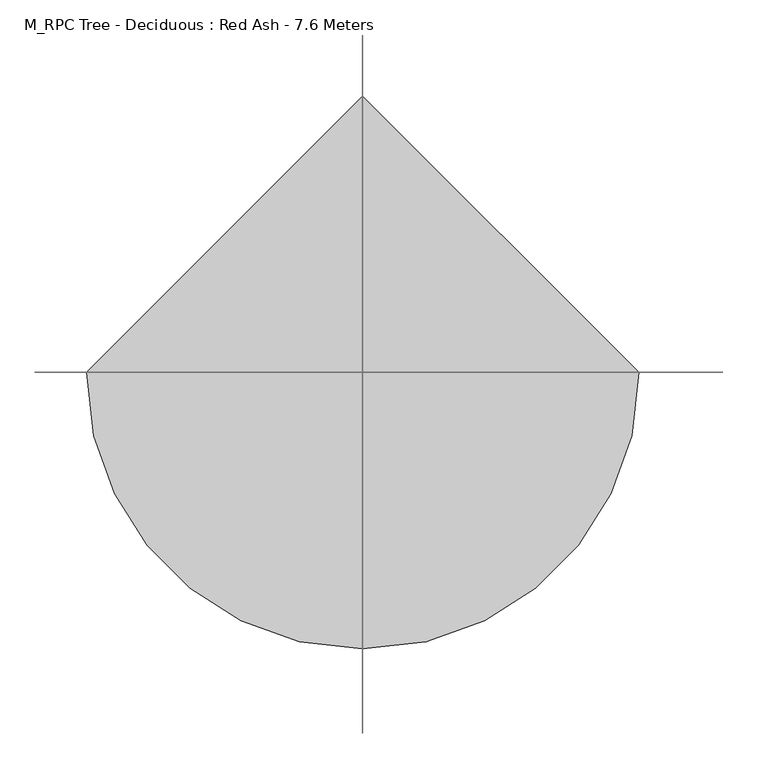
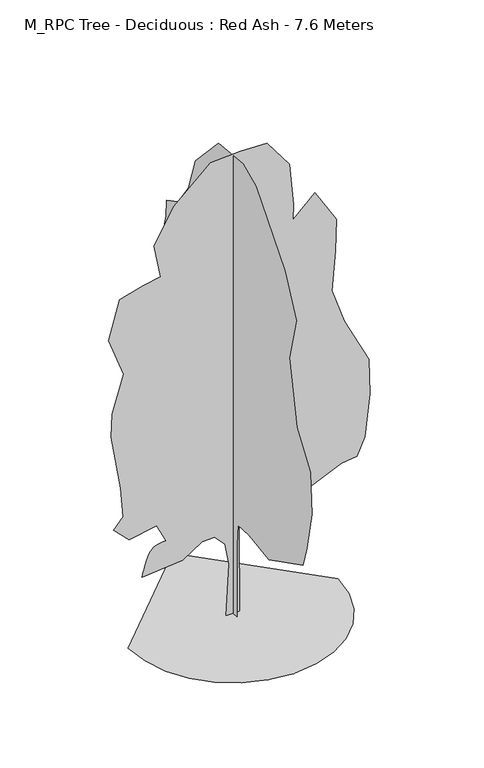
"""IFC4 building model written with IfcOpenShell, lengths in millimetres: geographic element geometry, M_RPC Tree - Deciduous : Red Ash - 7.6 Meters."""

import ifcopenshell
import ifcopenshell.guid

model = None  # the IFC model being written
_history = None  # IfcOwnerHistory: only IFC2X3 demands one
_inside = {}  # id of a spatial element -> (the spatial element, [elements in it])
_under = {}  # id of a project, library or spatial element -> (it, [spatial elements below it])
_declared = {}  # id of a project -> (the project, [libraries it declares])
_typed = {}  # id of a type object -> (the type object, [elements of that type])
_made_of = {}  # id of a material, layer set ... -> (it, [elements and type objects made of it])


def new_model(schema):
    """Start an empty IFC model of exactly this schema.

    Asked for "IFC4X3", IfcOpenShell would pick the latest addendum, in which some entities
    have other attributes; the version numbers below select the first issue.
    IFC2X3 requires an IfcOwnerHistory on every rooted entity: one is made here for all.
    """
    global model, _history
    if schema == "IFC4X3":
        model = ifcopenshell.file(schema_version=(4, 3, 0, 0))
    else:
        model = ifcopenshell.file(schema=schema)
    _inside.clear()
    _under.clear()
    _declared.clear()
    _typed.clear()
    _made_of.clear()
    _history = None
    if model.schema == "IFC2X3":
        org = make("IfcOrganization", Name="unknown")
        user = make(
            "IfcPersonAndOrganization",
            ThePerson=make("IfcPerson", FamilyName="unknown"),
            TheOrganization=org,
        )
        app = make(
            "IfcApplication",
            ApplicationDeveloper=org,
            Version="unknown",
            ApplicationFullName="unknown",
            ApplicationIdentifier="unknown",
        )
        _history = make(
            "IfcOwnerHistory",
            OwningUser=user,
            OwningApplication=app,
            ChangeAction="ADDED",
            CreationDate=0,
        )
    return model


def make(cls, **values):
    """One entity of the class cls with the attributes given. An attribute that is None is left unset."""
    return model.create_entity(
        cls, **{name: value for name, value in values.items() if value is not None}
    )


def rooted(cls, **values):
    """An entity with a GlobalId (a new one), such as an element, a storey or a relation."""
    return make(cls, GlobalId=ifcopenshell.guid.new(), OwnerHistory=_history, **values)


def si_unit(unit_type, name, prefix=None):
    """IfcSIUnit, for example si_unit("LENGTHUNIT", "METRE", prefix="MILLI")."""
    return make("IfcSIUnit", UnitType=unit_type, Prefix=prefix, Name=name)


def assignment(units):
    """IfcUnitAssignment: the units of a project."""
    return None if units is None else make("IfcUnitAssignment", Units=units)


def point(xyz):
    """IfcCartesianPoint."""
    return None if xyz is None else make("IfcCartesianPoint", Coordinates=xyz)


def direction(xyz):
    """IfcDirection."""
    return None if xyz is None else make("IfcDirection", DirectionRatios=xyz)


def frame(location, z_axis=None, x_axis=None):
    """IfcAxis2Placement3D, a coordinate frame: its origin and axes. An axis left out is left unset."""
    return make(
        "IfcAxis2Placement3D",
        Location=point(location),
        Axis=direction(z_axis),
        RefDirection=direction(x_axis),
    )


def origin():
    """The frame at (0, 0, 0) with its axes left unset."""
    return frame((0.0, 0.0, 0.0))


def place(relative_to, where):
    """IfcLocalPlacement: puts the frame where relative to a parent placement (None: the world)."""
    return make(
        "IfcLocalPlacement", PlacementRelTo=relative_to, RelativePlacement=where
    )


def context(
    kind, dimensions, precision=None, world=None, true_north=None, identifier=None
):
    """IfcGeometricRepresentationContext, for example the 3D "Model" context."""
    return make(
        "IfcGeometricRepresentationContext",
        ContextIdentifier=identifier,
        ContextType=kind,
        CoordinateSpaceDimension=dimensions,
        Precision=precision,
        WorldCoordinateSystem=world,
        TrueNorth=true_north,
    )


def project(units=None, contexts=None):
    """IfcProject with its units and contexts."""
    return rooted(
        "IfcProject",
        Name="project",
        RepresentationContexts=contexts,
        UnitsInContext=assignment(units),
    )


def spatial(cls, under=None, at=None, **own):
    """A site, building, storey or space (cls), placed at a placement, below another one or the project."""
    s = rooted(cls, ObjectPlacement=at, **own)
    if under is not None:
        _under.setdefault(under.id(), (under, []))[1].append(s)
    return s


def point_list(points):
    """IfcCartesianPointList2D or 3D."""
    cls = (
        "IfcCartesianPointList2D" if len(points[0]) == 2 else "IfcCartesianPointList3D"
    )
    return make(cls, CoordList=points)


def triangles(points, corners, closed=None, point_numbers=None):
    """IfcTriangulatedFaceSet: each triangle names its three corners, points numbered from 1."""
    return make(
        "IfcTriangulatedFaceSet",
        Coordinates=point_list(points),
        Closed=closed,
        CoordIndex=corners,
        PnIndex=point_numbers,
    )


def shape(context_of_items, identifier, shape_type, items):
    """IfcShapeRepresentation: the items that make up one representation, for example the "Body"."""
    return make(
        "IfcShapeRepresentation",
        ContextOfItems=context_of_items,
        RepresentationIdentifier=identifier,
        RepresentationType=shape_type,
        Items=items,
    )


def source(mapping_origin, context_of_items, identifier, shape_type, items):
    """IfcRepresentationMap: a shape defined once, which mapped items show again and again."""
    return make(
        "IfcRepresentationMap",
        MappingOrigin=mapping_origin,
        MappedRepresentation=shape(context_of_items, identifier, shape_type, items),
    )


def transform(
    local_origin,
    x_axis=None,
    y_axis=None,
    z_axis=None,
    scale=None,
    scale2=None,
    scale3=None,
    uniform=True,
):
    """IfcCartesianTransformationOperator3D, or its non-uniform kind. x_axis, y_axis, z_axis: its Axis1, 2, 3."""
    if uniform:
        return make(
            "IfcCartesianTransformationOperator3D",
            Axis1=direction(x_axis),
            Axis2=direction(y_axis),
            LocalOrigin=point(local_origin),
            Scale=scale,
            Axis3=direction(z_axis),
        )
    return make(
        "IfcCartesianTransformationOperator3DnonUniform",
        Axis1=direction(x_axis),
        Axis2=direction(y_axis),
        LocalOrigin=point(local_origin),
        Scale=scale,
        Axis3=direction(z_axis),
        Scale2=scale2,
        Scale3=scale3,
    )


def mapped(mapping_source, mapping_target):
    """IfcMappedItem: shows the shape of a source again, moved by a transform."""
    return make(
        "IfcMappedItem", MappingSource=mapping_source, MappingTarget=mapping_target
    )


def made_of(thing, what):
    """Note that an element or type object is made of a material, layer set ...; save() writes the relation."""
    if what is not None:
        _made_of.setdefault(what.id(), (what, []))[1].append(thing)
    return thing


def element(
    cls,
    number,
    at=None,
    inside=None,
    cuts=None,
    type_object=None,
    material=None,
    context=None,
    identifier="Body",
    shape_type=None,
    held_by="IfcProductDefinitionShape",
    body=None,
    shapes=None,
    **own,
):
    """One element of the class cls, such as IfcWall. Its Tag is "e" and its number.

    at: its placement. inside: the storey or other place that contains it. cuts: it is an
    opening in that element (IfcRelVoidsElement). A single representation is given by context,
    identifier, shape_type and body (its items); several are given by shapes. held_by: the class
    of the entity that holds the representations. save() writes the other relations.
    """
    e = rooted(cls, Tag="e%d" % number, ObjectPlacement=at, **own)
    if body is not None:
        shapes = [shape(context, identifier, shape_type, body)]
    if shapes is not None:
        e.Representation = make(held_by, Representations=shapes)
    if inside is not None:
        _inside.setdefault(inside.id(), (inside, []))[1].append(e)
    if cuts is not None:
        rooted(
            "IfcRelVoidsElement", RelatingBuildingElement=cuts, RelatedOpeningElement=e
        )
    if type_object is not None:
        _typed.setdefault(type_object.id(), (type_object, []))[1].append(e)
    return made_of(e, material)


def aggregate(whole, parts):
    """IfcRelAggregates: a whole, such as a stair, and the parts it consists of."""
    return rooted("IfcRelAggregates", RelatingObject=whole, RelatedObjects=parts)


def save(model, path):
    """Write the relations noted so far, then the file.

    IfcRelAggregates (storeys below a building ...), IfcRelContainedInSpatialStructure (elements
    in a storey), IfcRelDefinesByType, IfcRelAssociatesMaterial and IfcRelDeclares: one each for
    every whole, place, type object, material and project.
    """
    for whole, parts in _under.values():
        aggregate(whole, parts)
    for where, things in _inside.values():
        rooted(
            "IfcRelContainedInSpatialStructure",
            RelatedElements=things,
            RelatingStructure=where,
        )
    for kind, things in _typed.values():
        rooted("IfcRelDefinesByType", RelatedObjects=things, RelatingType=kind)
    for what, things in _made_of.values():
        rooted("IfcRelAssociatesMaterial", RelatedObjects=things, RelatingMaterial=what)
    for by, libraries in _declared.values():
        rooted("IfcRelDeclares", RelatingContext=by, RelatedDefinitions=libraries)
    model.write(path)


def m_rpc_tree_deciduous_red_ash_7_6_meters_16c8020d(model_context):
    return source(origin(), model_context, "Body", "Tessellation", [
        triangles([(-1640.6350319, 0.0, 6.17e-05), (-1597.2618073, -375.9250554, 6.17e-05), (-1473.7362076, -721.1521299, 6.17e-05), (-1279.9481815, -1025.7899305, 6.17e-05), (-1025.7900759, -1279.9483269, 6.17e-05), (-721.1519119, -1473.7357716, 6.17e-05), (-375.9249101, -1597.2618073, 6.17e-05), (7.17e-05, -1640.6350319, 6.17e-05), (375.9250917, -1597.2619526, 6.17e-05), (721.1521299, -1473.7360622, 6.17e-05), (1025.7900759, -1279.9481815, 6.17e-05), (1279.9486176, -1025.7900759, 6.17e-05), (1473.7359169, -721.1518393, 6.17e-05), (1597.2618073, -375.9248011, 6.17e-05), (1640.6350319, 0.0001434, 6.17e-05), (-0.0002151, 1640.6350319, 6.17e-05), (-1.07e-05, -102.5763152, 0.0), (2.5e-05, -100.9809819, 1191.4187742), (3.22e-05, -129.5410573, 1533.7667004), (7e-07, -437.6736119, 1554.0757805), (-5.76e-05, -973.8285673, 1474.4268631), (-0.0001401, -1898.6961697, 1943.5624718), (-0.0001409, -2005.9272697, 2292.063438), (-0.0001357, -2139.9660358, 2935.4493118), (-0.0001116, -2099.7546822, 3605.6435783), (-5.8e-05, -1735.814106, 4130.1484818), (-5.5e-06, -1523.3897175, 5147.0898972), (-3.5e-06, -1711.0423622, 5870.899205), (4.78e-05, -1402.7536217, 6514.2855148), (0.0001565, -625.3287638, 7439.1534805), (0.000198, -272.4836404, 7598.1990051), (0.0002655, 393.3664327, 7532.9808929), (0.0003113, 1023.3488731, 6862.7869171), (0.0003141, 1211.0034073, 6299.8236053), (0.0003314, 1492.4837551, 5897.706871), (0.0003588, 1800.7742397, 5736.8608749), (0.0003522, 1814.1780727, 5468.7830521), (0.0003514, 1894.6015068, 5160.4937302), (0.0003267, 1760.5627407, 4798.5890762), (0.0003288, 1881.1975285, 4450.088546), (0.000327, 2001.8324615, 3967.5488136), (0.0003203, 1975.0247955, 3833.5096115), (0.0002869, 1747.159053, 3511.8164566), (0.0002722, 1732.7516476, 3069.4885139), (0.0002625, 1720.3510963, 2788.0068581), (0.0002535, 1733.7549294, 2439.5063278), (0.0002406, 1747.159053, 1956.9668861), (0.0002166, 1559.5045189, 1809.523851), (0.0001802, 1211.0038433, 1809.523851), (0.0001822, 1371.8504208, 1313.580431), (0.0001711, 1344.9556961, 1032.1683203), (0.0001512, 1100.1359739, 1224.6137684), (9.84e-05, 627.810589, 1103.8028286), (9.77e-05, 550.2637599, 1353.49907), (6.27e-05, 215.346067, 1350.4488201), (5.01e-05, 130.4579254, 1225.1105404), (3.26e-05, 79.3405423, 816.1354311), (1.17e-05, 111.8716144, 1.28e-05), (-110.5798692, 4.8e-06, 4.45e-05), (-66.5363775, -9.62e-05, 831.3140104), (-128.9679092, -0.0001356, 1184.825572), (-290.0246482, -0.0001497, 1361.7341778), (-482.3670685, -0.0001405, 1355.1302204), (-794.1778324, -0.0001027, 1152.7338535), (-1424.1601639, -6.88e-05, 1099.1184488), (-1415.4458702, -7.33e-05, 1133.7810133), (-1406.1451298, -7.8e-05, 1169.6158899), (-1395.6722225, -8.3e-05, 1207.7952456), (-1383.4407017, -8.85e-05, 1249.4921917), (-1368.8645565, -9.46e-05, 1295.8774418), (-1351.3574856, -0.0001016, 1348.1257061), (-1330.3333328, -0.0001096, 1407.4074074), (-1303.8382931, -0.0001173, 1462.3908245), (-1271.0123898, -0.0001236, 1502.6024689), (-1232.9109364, -0.0001286, 1530.5039635), (-1190.588883, -0.0001326, 1548.5586754), (-1145.1018339, -0.0001358, 1559.2267742), (-1097.5041578, -0.0001386, 1564.971191), (-1048.8515316, -0.0001411, 1568.2539848), (-1196.294058, -0.0001698, 1863.1393284), (-1625.218531, -0.0001415, 1782.7160397), (-1866.4879612, -0.0001597, 2023.9861965), (-1719.0452168, -0.0001869, 2198.236607), (-1759.2568611, -0.0002427, 2680.7764847), (-1906.6994602, -0.0003433, 3578.8359123), (-1893.4979404, -0.0003882, 3950.7687332), (-1715.4032879, -0.0004676, 4551.3483536), (-1946.9112499, -0.0005333, 5187.3013962), (-1772.6605488, -0.0006144, 5803.88004), (-1410.7561855, -0.000643, 5911.1112854), (-1135.4252443, -0.0006608, 5959.6792511), (-1236.5059204, -0.0007209, 6500.8816818), (-928.2163805, -0.0007999, 7050.4411606), (-351.8493811, -0.0008874, 7573.192392), (117.2860368, -0.0009111, 7600.000058), (532.8066133, -0.0009277, 7586.5956436), (881.3074705, -0.000887, 7117.4603256), (945.3842279, -0.0008079, 6430.5952744), (936.1832634, -0.0007775, 6178.7100677), (1283.4236961, -0.0008311, 6500.8816818), (1618.5208294, -0.0007802, 5951.3222031), (1605.1169964, -0.0007177, 5432.2143539), (1545.3907001, -0.0006383, 4788.0519287), (1739.1557625, -0.0005793, 4222.2222221), (2126.1689129, -0.0005054, 3460.0925789), (2138.5076946, -0.0004374, 2885.2169128), (2060.8486267, -0.0003521, 2198.2364616), (1940.213839, -0.0003133, 1916.7548058), (1698.9439728, -0.0002996, 1889.9471397), (1229.8082188, -0.0002535, 1675.4849396), (814.2876514, -0.0002002, 1380.5997414), (256.8007496, -0.0002044, 1620.3048775), (92.8066444, -0.0001762, 1443.8352711), (103.8818677, -4.5e-06, 3.51e-05)], [[15, 16, 1], [14, 15, 1], [14, 1, 2], [13, 14, 2], [13, 2, 3], [13, 3, 4], [12, 13, 4], [11, 12, 4], [11, 4, 5], [11, 5, 6], [11, 6, 7], [11, 7, 8], [11, 8, 9], [11, 9, 10], [50, 51, 52], [57, 58, 17], [57, 17, 18], [56, 57, 18], [56, 18, 19], [55, 56, 19], [49, 50, 52], [52, 53, 54], [49, 52, 54], [35, 36, 37], [46, 47, 48], [46, 48, 49], [21, 22, 23], [20, 21, 23], [20, 23, 24], [20, 24, 25], [20, 25, 26], [19, 20, 26], [19, 26, 27], [45, 46, 49], [31, 32, 33], [30, 31, 33], [29, 30, 33], [29, 33, 34], [28, 29, 34], [27, 28, 34], [19, 27, 34], [19, 34, 35], [19, 35, 37], [19, 37, 38], [19, 38, 39], [19, 39, 40], [19, 40, 41], [19, 41, 42], [19, 42, 43], [19, 43, 44], [19, 44, 45], [19, 45, 49], [19, 49, 54], [55, 19, 54], [64, 65, 66], [64, 66, 67], [64, 67, 68], [99, 100, 101], [64, 68, 69], [64, 69, 70], [64, 70, 71], [114, 59, 60], [113, 114, 60], [113, 60, 61], [113, 61, 62], [64, 71, 72], [64, 72, 73], [64, 73, 74], [64, 74, 75], [64, 75, 76], [64, 76, 77], [64, 77, 78], [64, 78, 79], [63, 64, 79], [81, 82, 83], [80, 81, 83], [99, 101, 102], [107, 108, 109], [110, 111, 112], [88, 89, 90], [87, 88, 90], [87, 90, 91], [80, 83, 84], [95, 96, 97], [95, 97, 98], [94, 95, 98], [93, 94, 98], [92, 93, 98], [91, 92, 98], [91, 98, 99], [87, 91, 99], [87, 99, 102], [87, 102, 103], [87, 103, 104], [86, 87, 104], [85, 86, 104], [84, 85, 104], [80, 84, 104], [80, 104, 105], [80, 105, 106], [80, 106, 107], [80, 107, 109], [80, 109, 110], [80, 110, 112], [79, 80, 112], [63, 79, 112], [62, 63, 112], [113, 62, 112]], closed=False),
    ])


if __name__ == "__main__":
    model = new_model("IFC4")
    model_context = context("Model", 3, world=origin())
    ifc_project = project(units=[si_unit("LENGTHUNIT", "METRE", prefix="MILLI")], contexts=[model_context])
    site = spatial("IfcSite", under=ifc_project)
    building = spatial("IfcBuilding", under=site)
    placement = place(None, origin())
    m_rpc_tree_deciduous_red_ash_7_6_meters_shape = m_rpc_tree_deciduous_red_ash_7_6_meters_16c8020d(model_context)
    element("IfcGeographicElement", 1, ObjectType="M_RPC Tree - Deciduous : Red Ash - 7.6 Meters", at=placement, inside=building, context=model_context, shape_type="MappedRepresentation", body=[
        mapped(m_rpc_tree_deciduous_red_ash_7_6_meters_shape, transform((0.0, 0.0, 0.0), x_axis=(1.0, 0.0, 0.0), y_axis=(0.0, 1.0, 0.0), z_axis=(0.0, 0.0, 1.0))),
    ])
    save(model, "model.ifc")

# Revit data of these elements
# Type "M_RPC Tree - Deciduous : Red Ash - 7.6 Meters"
#   built-in parameter 1005198 = "{2, 15},{22, RPC-8-G3GR-497X-PHW5-6},{1, 0},{1, 0},{2, 37},{1, 8},{5, Color},{1, 0},{1, 0},{3, 0.8},{3, 0.8},{3, 0.8},{1, 8},{7, BBoxMin},{1, 0},{1, 0},{1, 0},{1, 0},{1, 0},{1, 8},{7, BBoxMax},{1, 0},{1, 0},{1, 0},{1, 0},{1, 0},{2, 11},{9, RPCTypeId},{1, 0},{1, 0},{22, RPC-8-G3GR-497X-PHW5-6},{1, 6},{14, RPCPlantHeight},{1, 0},{1, 0},{7, 24.9344},{2, 11},{7, keyword},{1, 0},{1, 0},{78, :Geometry:RPC:Red Ash:red ash:frainus pennsylvanica:frene rouge:deciduous:tree},{2, 11},{8, category},{1, 0},{1, 0},{16, :Trees [General]},{2, 11},{12, LocalizedUID},{1, 0},{1, 0},{7, Red Ash},{2, 14},{6, Height},{1, 0},{1, 0},{7, 24.9344},{1, 2},{16, Cast Reflections},{1, 0},{1, 0},{1, 0},{1, 2},{6, Jitter},{1, 0},{1, 0},{1, 1},{1, 2},{9, Billboard},{1, 0},{1, 0},{1, 0},{1, 2},{12, Cast Shadows},{1, 0},{1, 0},{1, 1},{1, 2},{20, Apply Filter Effects},{1, 0},{1, 0},{1, 0},{2, 11},{28, Apply Filter Effects-Text-FC},{1, 0},{1, 0},{4, None},{2, 11},{20, AdvancedUIDefinition},{1, 0},{1, 0},{0, },{2, 11},{10, AssetLibID},{1, 0},{1, 0},{36, 4D3F6E72-3F99-4203-98E9-AF80B3C7A7A4},{2, 11},{10, BaseSchema},{1, 0},{1, 0},{9, RPCSchema},{2, 11},{12, ExchangeGUID},{1, 0},{1, 0},{0, },{1, 2},{6, Hidden},{1, 0},{1, 0},{1, 0},{1, 4},{11, RPCCategory},{1, 0},{1, 0},{1, 0},{2, 11},{8, RPCImage},{1, 0},{1, 0},{0, },{1, 4},{13, SchemaVersion},{1, 0},{1, 0},{1, 4},{2, 11},{12, UIDefinition},{1, 0},{1, 0},{0, },{2, 11},{6, UIName},{1, 0},{1, 0},{22, RPC-8-G3GR-497X-PHW5-6},{2, 11},{11, VersionGUID},{1, 0},{1, 0},{9, RPCSchema},{2, 11},{9, assettype},{1, 0},{1, 0},{11, RPCGeometry},{2, 11},{11, description},{1, 0},{1, 0},{0, },{2, 11},{9, localname},{1, 0},{1, 0},{3, RPC},{2, 11},{9, localtype},{1, 0},{1, 0},{3, RPC},{1, 4},{8, revision},{1, 0},{1, 0},{1, 1},{2, 11},{9, thumbnail},{1, 0},{1, 0},{0, },{1, 4},{7, version},{1, 0},{1, 0},{1, 1},{1, 2},{20, RPC_Cast Reflections},{1, 0},{1, 0},{1, 1},{1, 2},{10, RPC_Jitter},{1, 0},{1, 0},{1, 1},{1, 2},{13, RPC_Billboard},{1, 0},{1, 0},{1, 0},{1, 2},{16, RPC_Cast Shadows},{1, 0},{1, 0},{1, 1},{21, assetlibrary_base.fbx},{1, 5},"
#   built-in parameter 1005195 = "RPC-8-G3GR-497X-PHW5-6"
#   Type Comments = "Red Ash"
#   Height = 7.60 m
#   Default Elevation = 0
